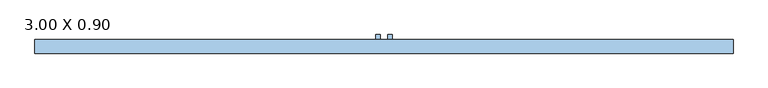
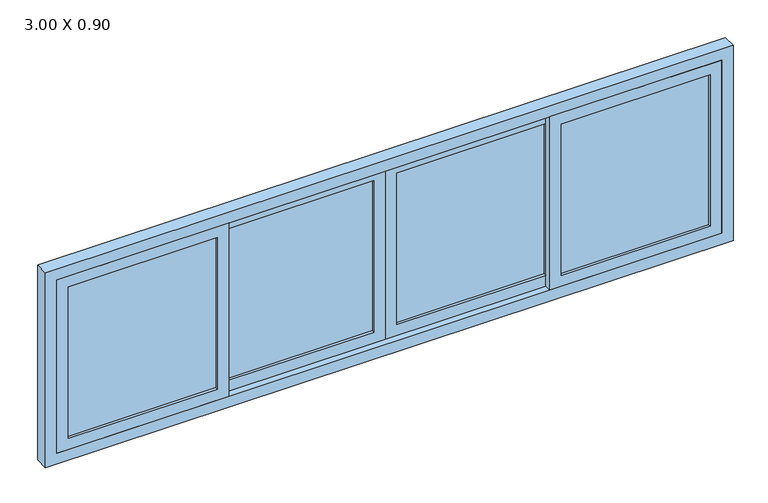
"""IFC4 building model written with IfcOpenShell, lengths in millimetres: window geometry, .CC_ND 300_JANELA_4 FOLHAS DE CORRER_VIDRO : 3.00 X 0.90."""

from ifc_helpers import new_model, si_unit, frame, origin, place, context, project, spatial, polyline, outline, extrude, source, transform, mapped, element, save


def window_3_00_x_0_90_5327f378(model_context):
    return source(origin(), model_context, "Body", "SweptSolid", [
        extrude(outline(polyline([(-50.0, 12.5), (-700.0, 12.5), (-700.0, 17.5), (-50.0, 17.5), (-50.0, 12.5)])), frame((0.0, 0.0, 1100.0), z_axis=(0.0, 0.0, 1.0), x_axis=(1.0, 0.0, 0.0)), (0.0, 0.0, 1.0), 700.0),
        extrude(outline(polyline([(1850.0, 0.0), (1850.0, -750.0), (1050.0, -750.0), (1050.0, 0.0), (1850.0, 0.0)]), holes=[polyline([(1800.0, -50.0), (1100.0, -50.0), (1100.0, -700.0), (1800.0, -700.0), (1800.0, -50.0)])]), frame((0.0, 0.0, 0.0), z_axis=(0.0, 1.0, 0.0), x_axis=(0.0, 0.0, 1.0)), (0.0, 0.0, 1.0), 30.0),
        extrude(outline(polyline([(-750.0, -17.5), (-1400.0, -17.5), (-1400.0, -12.5), (-750.0, -12.5), (-750.0, -17.5)])), frame((0.0, 0.0, 1100.0), z_axis=(0.0, 0.0, 1.0), x_axis=(1.0, 0.0, 0.0)), (0.0, 0.0, 1.0), 700.0),
        extrude(outline(polyline([(1850.0, -700.0), (1850.0, -1450.0), (1050.0, -1450.0), (1050.0, -700.0), (1850.0, -700.0)]), holes=[polyline([(1800.0, -750.0), (1100.0, -750.0), (1100.0, -1400.0), (1800.0, -1400.0), (1800.0, -750.0)])]), frame((0.0, -30.0, 0.0), z_axis=(0.0, 1.0, 0.0), x_axis=(0.0, 0.0, 1.0)), (0.0, 0.0, 1.0), 30.0),
        extrude(outline(polyline([(1400.0, -17.5), (750.0, -17.5), (750.0, -12.5), (1400.0, -12.5), (1400.0, -17.5)])), frame((0.0, 0.0, 1100.0), z_axis=(0.0, 0.0, 1.0), x_axis=(1.0, 0.0, 0.0)), (0.0, 0.0, 1.0), 700.0),
        extrude(outline(polyline([(1850.0, 1450.0), (1850.0, 700.0), (1050.0, 700.0), (1050.0, 1450.0), (1850.0, 1450.0)]), holes=[polyline([(1800.0, 1400.0), (1100.0, 1400.0), (1100.0, 750.0), (1800.0, 750.0), (1800.0, 1400.0)])]), frame((0.0, -30.0, 0.0), z_axis=(0.0, 1.0, 0.0), x_axis=(0.0, 0.0, 1.0)), (0.0, 0.0, 1.0), 30.0),
        extrude(outline(polyline([(700.0, 12.5), (50.0, 12.5), (50.0, 17.5), (700.0, 17.5), (700.0, 12.5)])), frame((0.0, 0.0, 1100.0), z_axis=(0.0, 0.0, 1.0), x_axis=(1.0, 0.0, 0.0)), (0.0, 0.0, 1.0), 700.0),
        extrude(outline(polyline([(1850.0, 750.0), (1850.0, 0.0), (1050.0, 0.0), (1050.0, 750.0), (1850.0, 750.0)]), holes=[polyline([(1800.0, 700.0), (1100.0, 700.0), (1100.0, 50.0), (1800.0, 50.0), (1800.0, 700.0)])]), frame((0.0, 0.0, 0.0), z_axis=(0.0, 1.0, 0.0), x_axis=(0.0, 0.0, 1.0)), (0.0, 0.0, 1.0), 30.0),
        extrude(outline(polyline([(1900.0, -1500.0), (1000.0, -1500.0), (1000.0, 1500.0), (1900.0, 1500.0), (1900.0, -1500.0)]), holes=[polyline([(1050.0, -1450.0), (1850.0, -1450.0), (1850.0, 1450.0), (1050.0, 1450.0), (1050.0, -1450.0)])]), frame((0.0, -30.0, 0.0), z_axis=(0.0, 1.0, 0.0), x_axis=(0.0, 0.0, 1.0)), (0.0, 0.0, 1.0), 60.0),
        extrude(outline(polyline([(-35.9492003, 30.0), (-35.9492003, 50.0), (-15.9492003, 50.0), (-15.9492003, 30.0), (-35.9492003, 30.0)])), frame((0.0, 0.0, 1390.0), z_axis=(0.0, 0.0, 1.0), x_axis=(1.0, 0.0, 0.0)), (0.0, 0.0, 1.0), 120.0),
        extrude(outline(polyline([(15.9492003, 30.0), (15.9492003, 50.0), (35.9492003, 50.0), (35.9492003, 30.0), (15.9492003, 30.0)])), frame((0.0, 0.0, 1390.0), z_axis=(0.0, 0.0, 1.0), x_axis=(1.0, 0.0, 0.0)), (0.0, 0.0, 1.0), 120.0),
    ])


if __name__ == "__main__":
    model = new_model("IFC4")
    model_context = context("Model", 3, world=origin())
    ifc_project = project(units=[si_unit("LENGTHUNIT", "METRE", prefix="MILLI")], contexts=[model_context])
    site = spatial("IfcSite", under=ifc_project)
    building = spatial("IfcBuilding", under=site)
    placement = place(None, origin())
    window_3_00_x_0_90_shape = window_3_00_x_0_90_5327f378(model_context)
    element("IfcWindow", 1, ObjectType=".CC_ND 300_JANELA_4 FOLHAS DE CORRER_VIDRO : 3.00 X 0.90", at=placement, inside=building, context=model_context, shape_type="MappedRepresentation", body=[
        mapped(window_3_00_x_0_90_shape, transform((0.0, 0.0, 0.0), x_axis=(1.0, 0.0, 0.0), y_axis=(0.0, 1.0, 0.0), z_axis=(0.0, 0.0, 1.0))),
    ])
    save(model, "model.ifc")

# Revit data of these elements
# Type ".CC_ND 300_JANELA_4 FOLHAS DE CORRER_VIDRO : 3.00 X 0.90"
#   Type Mark = "61"
#   Largura moldura = 0.06 m
#   Largura janela = 2.90 m
#   Largura esquadria = 0.05 m
#   Largura do painel = 0.75 m
#   Largura da moldura do painel = 0.05 m
#   Espessura painel = 0.03 m
#   Espessura moldura = 0.03 m
#   Altura janela = 0.80 m
#   Height = 0.90 m
#   Altura-padrão do peitoril = 1.00 m
#   Width = 3.00 m
#   Puxadores [instance default] = yes
#   Moldura interna [instance default] = yes
#   Moldura externa [instance default] = yes
#   Tipo de vidro = .VIDRO GENÉRICO
#   Material puxadores = .ALUMÍNIO COM PINTURA ELETROSTÁTICA BRANCA
#   Material moldura = .ALUMÍNIO COM PINTURA ELETROSTÁTICA BRANCA
#   Material da esquadria = .ALUMÍNIO COM PINTURA ELETROSTÁTICA BRANCA
#   Wall Closure = (empty or 0)
# Element 1 (IfcWindow, ".CC_ND 300_JANELA_4 FOLHAS DE CORRER_VIDRO : 3.00 X 0.90")
#   Moldura interna = no
#   Moldura externa = no
#   Materials on its faces: ".ALUMÍNIO COM PINTURA ELETROSTÁTICA BRANCA", ".VIDRO GENÉRICO"
# Materials
#   ".VIDRO GENÉRICO": class ".CC_VIDRO", colour RGB 0 128 192, transparency 0.9, Description = "Vidro comum", Cost = 0
#   ".ALUMÍNIO COM PINTURA ELETROSTÁTICA BRANCA": class "CC_METAIS", colour RGB 241 241 241, transparency 0, Cost = 0
